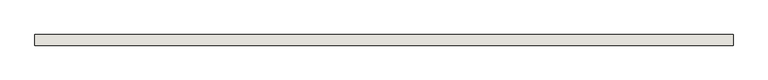
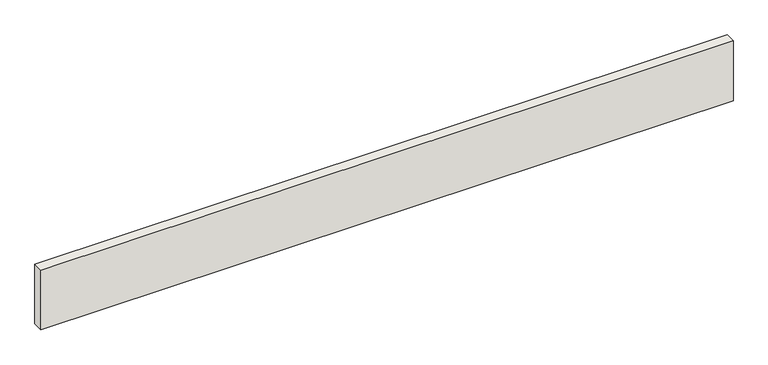
"""IFC4 building model written with IfcOpenShell, lengths in millimetres: wall geometry, Holzwand."""

from ifc_helpers import new_model, si_unit, origin, origin_with_axes, place, context, project, spatial, polyline, outline, extrude, source, transform, mapped, element, save


def wall_864364e1(model_context):
    return source(origin(), model_context, "Body", "SweptSolid", [
        extrude(outline(polyline([(13165.5042912, 200.0), (13165.5042912, 0.0), (0.0, 0.0), (0.0, 200.0), (13165.5042912, 200.0)])), origin_with_axes(), (0.0, 0.0, 1.0), 1200.0),
    ])


if __name__ == "__main__":
    model = new_model("IFC4")
    model_context = context("Model", 3, world=origin())
    ifc_project = project(units=[si_unit("LENGTHUNIT", "METRE", prefix="MILLI")], contexts=[model_context])
    site = spatial("IfcSite", under=ifc_project)
    building = spatial("IfcBuilding", under=site)
    placement = place(None, origin())
    wall_shape = wall_864364e1(model_context)
    element("IfcWall", 1, ObjectType="Holzwand", at=placement, inside=building, context=model_context, shape_type="MappedRepresentation", body=[
        mapped(wall_shape, transform((0.0, 0.0, 0.0), x_axis=(1.0, 0.0, 0.0), y_axis=(0.0, 1.0, 0.0), z_axis=(0.0, 0.0, 1.0))),
    ])
    save(model, "model.ifc")

# Revit data of these elements
# Element 1 (IfcWall, "Holzwand")
#   Materials on its faces: "NC-GK-Platte-grau"
# Materials
#   "NC-GK-Platte-grau": class "Unassigned", colour RGB 199 199 199, transparency 0
